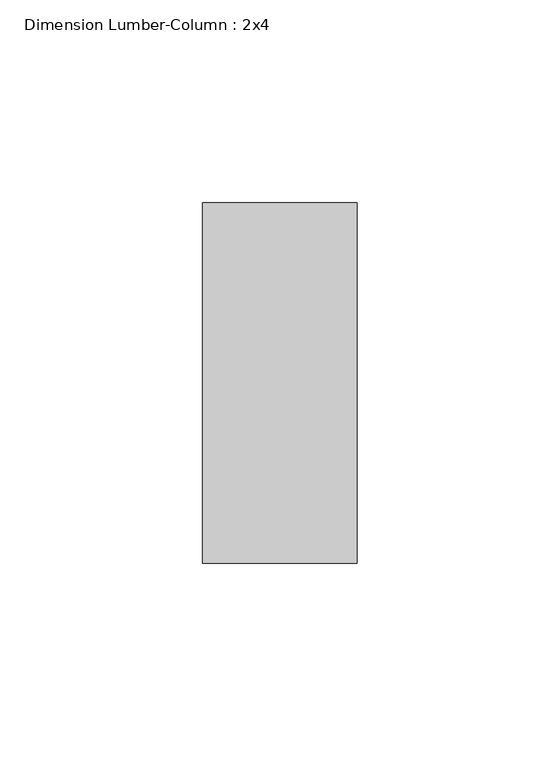
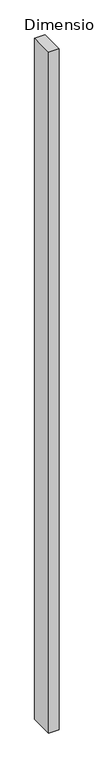
"""IFC4 building model written with IfcOpenShell, lengths in millimetres: column geometry, Dimension Lumber-Column : 2x4."""

from ifc_helpers import new_model, si_unit, frame, origin, place, context, project, spatial, polyline, outline, extrude, source, transform, mapped, element, save


def dimension_lumber_column_2x4_07183c39(model_context):
    return source(origin(), model_context, "Body", "SweptSolid", [
        extrude(outline(polyline([(19.05, 44.45), (19.05, -44.45), (-19.05, -44.45), (-19.05, 44.45), (19.05, 44.45)])), frame((0.0, 0.0, 56.35625), z_axis=(0.0, 0.0, 1.0), x_axis=(1.0, 0.0, 0.0)), (0.0, 0.0, 1.0), 2636.04375),
    ])


if __name__ == "__main__":
    model = new_model("IFC4")
    model_context = context("Model", 3, world=origin())
    ifc_project = project(units=[si_unit("LENGTHUNIT", "METRE", prefix="MILLI")], contexts=[model_context])
    site = spatial("IfcSite", under=ifc_project)
    building = spatial("IfcBuilding", under=site)
    placement = place(None, origin())
    dimension_lumber_column_2x4_shape = dimension_lumber_column_2x4_07183c39(model_context)
    element("IfcColumn", 1, ObjectType="Dimension Lumber-Column : 2x4", at=placement, inside=building, context=model_context, shape_type="MappedRepresentation", body=[
        mapped(dimension_lumber_column_2x4_shape, transform((0.0, 0.0, 0.0), x_axis=(1.0, 0.0, 0.0), y_axis=(0.0, 1.0, 0.0), z_axis=(0.0, 0.0, 1.0))),
    ])
    save(model, "model.ifc")

# Revit data of these elements
# Type "Dimension Lumber-Column : 2x4"
#   Int Type = "Interior"
#   Assembly Code = "B10"
#   Cost = 8.05
#   A = 0.0364583 SF
#   b = 0' - 1 1/2"
#   d = 0' - 3 1/2"
#   Structural Material [instance default] = Softwood, Lumber
# Element 1 (IfcColumn, "Dimension Lumber-Column : 2x4")
#   Structural Material = Douglas Fir #2
#   Materials on its faces: "Douglas Fir #2"
# Materials
#   "Softwood, Lumber": class "Wood", colour RGB 223 192 134, transparency 0, Description = "Pinus Echinata", Cost = 0
#   "Douglas Fir #2": class "Wood", colour RGB 223 192 134, transparency 0, Description = "Pinus Echinata", Cost = 0
